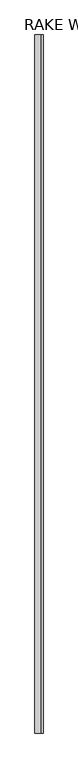
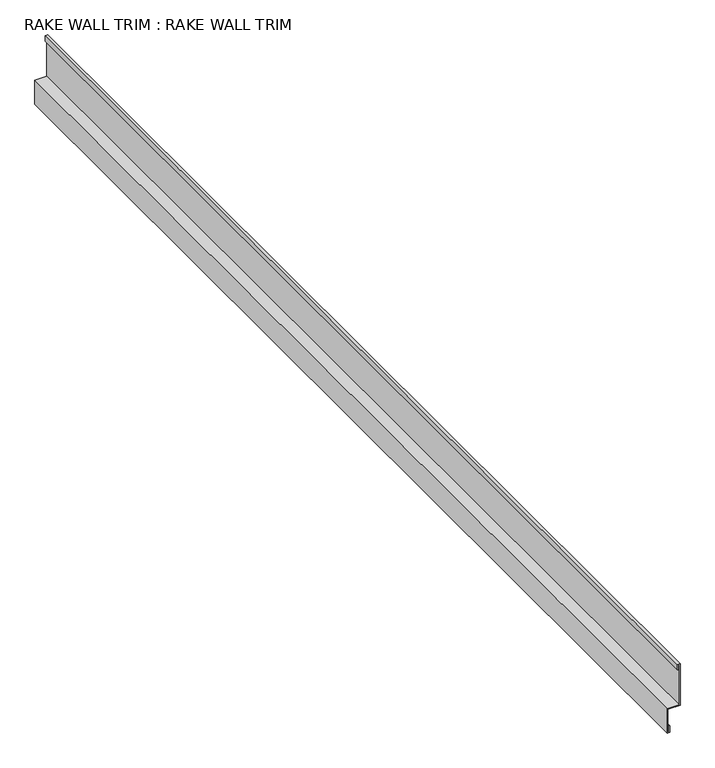
"""IFC4 building model written with IfcOpenShell, lengths in millimetres: proxy geometry, RAKE WALL TRIM : RAKE WALL TRIM."""

from ifc_helpers import new_model, si_unit, frame, origin, place, context, project, spatial, polyline, outline, extrude, source, transform, mapped, element, save


def rake_wall_trim_rake_wall_trim_6c46a03a(model_context):
    return source(origin(), model_context, "Body", "SweptSolid", [
        extrude(outline(polyline([(42587.6891059, 6031.9273326), (42600.6594931, 6031.9273326), (42600.6594931, 6030.7367076), (42588.8797309, 6030.7367076), (42588.8797309, 6029.0648149), (42633.0181981, 6029.0648149), (42633.0181981, 6051.059243), (42713.3823263, 6051.059243), (42713.3823263, 6046.3607241), (42703.1990698, 6046.3607241), (42703.1990698, 6047.5513491), (42712.1917013, 6047.5513491), (42712.1917013, 6049.868618), (42634.2088231, 6049.868618), (42634.2088231, 6027.8741899), (42587.6891059, 6027.8741899), (42587.6891059, 6031.9273326)])), frame((0.0, -1052.8906574, 0.0), z_axis=(0.0, 1.0, 0.0), x_axis=(0.0, 0.0, 1.0)), (0.0, 0.0, 1.0), 1999.85),
    ])


if __name__ == "__main__":
    model = new_model("IFC4")
    model_context = context("Model", 3, world=origin())
    ifc_project = project(units=[si_unit("LENGTHUNIT", "METRE", prefix="MILLI")], contexts=[model_context])
    site = spatial("IfcSite", under=ifc_project)
    building = spatial("IfcBuilding", under=site)
    placement = place(None, origin())
    rake_wall_trim_rake_wall_trim_shape = rake_wall_trim_rake_wall_trim_6c46a03a(model_context)
    element("IfcBuildingElementProxy", 1, Name="RAKE WALL TRIM : RAKE WALL TRIM", ObjectType="RAKE WALL TRIM : RAKE WALL TRIM", at=placement, inside=building, context=model_context, shape_type="MappedRepresentation", body=[
        mapped(rake_wall_trim_rake_wall_trim_shape, transform((0.0, 0.0, 0.0), x_axis=(1.0, 0.0, 0.0), y_axis=(0.0, 1.0, 0.0), z_axis=(0.0, 0.0, 1.0))),
    ])
    save(model, "model.ifc")

# Revit data of these elements
# Type "RAKE WALL TRIM : RAKE WALL TRIM"
#   NameOverride = "RAKE WALL TRIM"
# Element 1 (IfcBuildingElementProxy, "RAKE WALL TRIM : RAKE WALL TRIM")
#   Materials on its faces: "RAKE WALL TRIM"
# Materials
#   "RAKE WALL TRIM": class "Unassigned", colour RGB 128 128 128, transparency 0, Cost = 0
